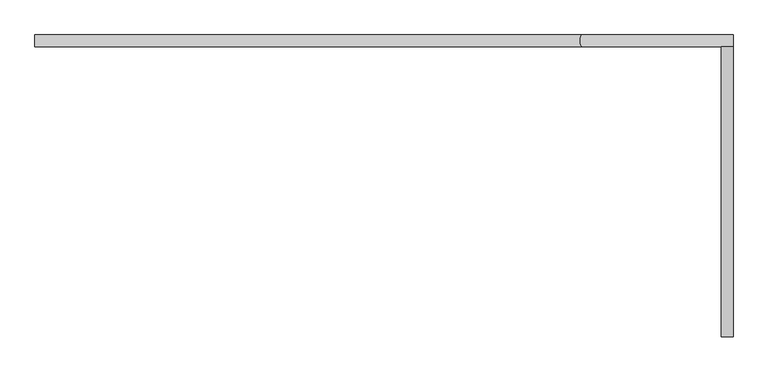
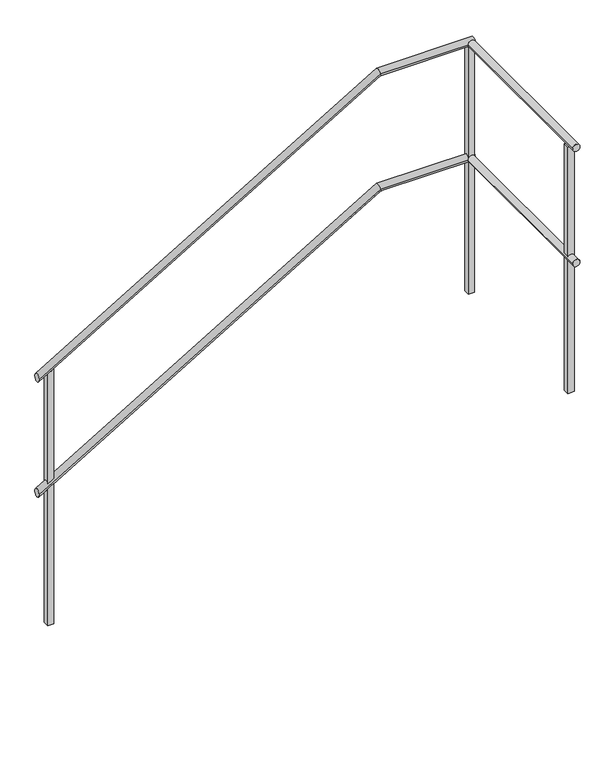
"""IFC4 building model written with IfcOpenShell, lengths in millimetres: railing geometry."""

from ifc_helpers import new_model, si_unit, frame, origin, place, context, project, spatial, polyline, circle_curve, ellipse_curve, outline, extrude, source, transform, mapped, element, save
from ifc_brep_helpers import plane_surface, cylinder_surface, advanced_brep


def railing_f6e22b08(model_context):
    return source(origin(), model_context, "Body", "SolidModel", [
        advanced_brep(
        [(43964.6, 23749.5208589, 1584.9618634), (43994.6, 23749.5208589, 1584.9618634), (43964.6, 24494.1208589, 1584.9618634), (43994.6, 24494.1208589, 1584.9618634)],
        [
            (0, 1, circle_curve(frame((43979.6, 23749.5208589, 1584.9618634), z_axis=(0.0, -1.0, 0.0), x_axis=(1.0, 0.0, 0.0)), 15.0)),
            (1, 0, circle_curve(frame((43979.6, 23749.5208589, 1584.9618634), z_axis=(0.0, -1.0, 0.0), x_axis=(1.0, 0.0, 0.0)), 15.0)),
            (2, 3, circle_curve(frame((43979.6, 24494.1208589, 1584.9618634), z_axis=(0.0, 1.0, 0.0), x_axis=(1.0, 0.0, 0.0)), 15.0)),
            (3, 2, circle_curve(frame((43979.6, 24494.1208589, 1584.9618634), z_axis=(0.0, 1.0, 0.0), x_axis=(1.0, 0.0, 0.0)), 15.0)),
            (0, 2),
            (3, 1),
        ],
        [
            plane_surface(frame((43979.6, 23749.5208589, 1599.9618634), z_axis=(0.0, -1.0, 0.0), x_axis=(0.0, 0.0, 1.0))),
            plane_surface(frame((43979.6, 24494.1208589, 1599.9618634), z_axis=(0.0, 1.0, 0.0), x_axis=(0.0, 0.0, 1.0))),
            cylinder_surface(frame((43979.6, 23749.5208589, 1584.9618634), z_axis=(0.0, -1.0, 0.0), x_axis=(1.0, 0.0, 0.0)), 15.0),
        ],
        [
            (0, [[1, 2]]),
            (1, [[3, 4]]),
            (2, [[-1, 5, -4, 6]]),
            (2, [[-2, -6, -3, -5]]),
        ],
    ),
        advanced_brep(
        [(43994.6, 24494.1208589, 1584.9618634), (43994.6, 24524.1208589, 1584.9618634), (43606.242552, 24494.1208589, 1584.9618634), (43606.242552, 24524.1208589, 1584.9618634), (42202.1161135, 24494.1208589, 749.1723166), (42202.1161135, 24524.1208589, 749.1723166)],
        [
            (0, 1, circle_curve(frame((43994.6, 24509.1208589, 1584.9618634), z_axis=(1.0, 0.0, 0.0), x_axis=(0.0, 1.0, 0.0)), 15.0)),
            (1, 0, circle_curve(frame((43994.6, 24509.1208589, 1584.9618634), z_axis=(1.0, 0.0, 0.0), x_axis=(0.0, 1.0, 0.0)), 15.0)),
            (0, 2),
            (2, 3, ellipse_curve(frame((43606.242552, 24509.1208589, 1584.9618634), z_axis=(0.9641817474962143, 0.0, 0.2652424509673111), x_axis=(0.265242450967311, 0.0, -0.9641817474962144)), 15.5572329, 15.0)),
            (3, 1),
            (3, 2, ellipse_curve(frame((43606.242552, 24509.1208589, 1584.9618634), z_axis=(0.9641817474962143, 0.0, 0.2652424509673111), x_axis=(0.265242450967311, 0.0, -0.9641817474962144)), 15.5572329, 15.0)),
            (4, 5, ellipse_curve(frame((42202.1161135, 24509.1208589, 749.1723166), z_axis=(-1.0, 0.0, 0.0), x_axis=(0.0, 0.0, 1.0)), 17.4562134, 15.0)),
            (5, 4, ellipse_curve(frame((42202.1161135, 24509.1208589, 749.1723166), z_axis=(-1.0, 0.0, 0.0), x_axis=(0.0, 0.0, 1.0)), 17.4562134, 15.0)),
            (2, 4),
            (5, 3),
        ],
        [
            plane_surface(frame((43994.6, 24509.1208589, 1599.9618634), z_axis=(1.0, 0.0, 0.0), x_axis=(0.0, -1.0, 0.0))),
            cylinder_surface(frame((43994.6, 24509.1208589, 1584.9618634), z_axis=(1.0, 0.0, 0.0), x_axis=(0.0, 1.0, 0.0)), 15.0),
            plane_surface(frame((42202.1161135, 24509.1208589, 766.62853), z_axis=(-1.0, 0.0, 0.0), x_axis=(0.0, -1.0, 0.0))),
            cylinder_surface(frame((43609.7883714, 24509.1208589, 1587.0724701), z_axis=(0.8592928844097072, 0.0, 0.5114838597676818), x_axis=(0.0, 1.0, 0.0)), 15.0),
        ],
        [
            (0, [[1, 2]]),
            (1, [[-1, 3, 4, 5]]),
            (1, [[-2, -5, 6, -3]]),
            (2, [[7, 8]]),
            (3, [[-4, 9, -8, 10]]),
            (3, [[-6, -10, -7, -9]]),
        ],
    ),
        advanced_brep(
        [(43964.6, 23749.5208589, 2084.9618634), (43994.6, 23749.5208589, 2084.9618634), (43964.6, 24494.1208589, 2084.9618634), (43994.6, 24494.1208589, 2084.9618634)],
        [
            (0, 1, circle_curve(frame((43979.6, 23749.5208589, 2084.9618634), z_axis=(0.0, -1.0, 0.0), x_axis=(1.0, 0.0, 0.0)), 15.0)),
            (1, 0, circle_curve(frame((43979.6, 23749.5208589, 2084.9618634), z_axis=(0.0, -1.0, 0.0), x_axis=(1.0, 0.0, 0.0)), 15.0)),
            (2, 3, circle_curve(frame((43979.6, 24494.1208589, 2084.9618634), z_axis=(0.0, 1.0, 0.0), x_axis=(1.0, 0.0, 0.0)), 15.0)),
            (3, 2, circle_curve(frame((43979.6, 24494.1208589, 2084.9618634), z_axis=(0.0, 1.0, 0.0), x_axis=(1.0, 0.0, 0.0)), 15.0)),
            (0, 2),
            (3, 1),
        ],
        [
            plane_surface(frame((43979.6, 23749.5208589, 2099.9618634), z_axis=(0.0, -1.0, 0.0), x_axis=(0.0, 0.0, 1.0))),
            plane_surface(frame((43979.6, 24494.1208589, 2099.9618634), z_axis=(0.0, 1.0, 0.0), x_axis=(0.0, 0.0, 1.0))),
            cylinder_surface(frame((43979.6, 23749.5208589, 2084.9618634), z_axis=(0.0, -1.0, 0.0), x_axis=(1.0, 0.0, 0.0)), 15.0),
        ],
        [
            (0, [[1, 2]]),
            (1, [[3, 4]]),
            (2, [[-1, 5, -4, 6]]),
            (2, [[-2, -6, -3, -5]]),
        ],
    ),
        advanced_brep(
        [(43994.6, 24494.1208589, 2084.9618634), (43994.6, 24524.1208589, 2084.9618634), (43606.242552, 24494.1208589, 2084.9618634), (43606.242552, 24524.1208589, 2084.9618634), (42202.1161135, 24494.1208589, 1249.1723166), (42202.1161135, 24524.1208589, 1249.1723166)],
        [
            (0, 1, circle_curve(frame((43994.6, 24509.1208589, 2084.9618634), z_axis=(1.0, 0.0, 0.0), x_axis=(0.0, 1.0, 0.0)), 15.0)),
            (1, 0, circle_curve(frame((43994.6, 24509.1208589, 2084.9618634), z_axis=(1.0, 0.0, 0.0), x_axis=(0.0, 1.0, 0.0)), 15.0)),
            (0, 2),
            (2, 3, ellipse_curve(frame((43606.242552, 24509.1208589, 2084.9618634), z_axis=(0.9641817474962143, 0.0, 0.2652424509673111), x_axis=(0.265242450967311, 0.0, -0.9641817474962144)), 15.5572329, 15.0)),
            (3, 1),
            (3, 2, ellipse_curve(frame((43606.242552, 24509.1208589, 2084.9618634), z_axis=(0.9641817474962143, 0.0, 0.2652424509673111), x_axis=(0.265242450967311, 0.0, -0.9641817474962144)), 15.5572329, 15.0)),
            (4, 5, ellipse_curve(frame((42202.1161135, 24509.1208589, 1249.1723166), z_axis=(-1.0, 0.0, 0.0), x_axis=(0.0, 0.0, 1.0)), 17.4562134, 15.0)),
            (5, 4, ellipse_curve(frame((42202.1161135, 24509.1208589, 1249.1723166), z_axis=(-1.0, 0.0, 0.0), x_axis=(0.0, 0.0, 1.0)), 17.4562134, 15.0)),
            (2, 4),
            (5, 3),
        ],
        [
            plane_surface(frame((43994.6, 24509.1208589, 2099.9618634), z_axis=(1.0, 0.0, 0.0), x_axis=(0.0, -1.0, 0.0))),
            cylinder_surface(frame((43994.6, 24509.1208589, 2084.9618634), z_axis=(1.0, 0.0, 0.0), x_axis=(0.0, 1.0, 0.0)), 15.0),
            plane_surface(frame((42202.1161135, 24509.1208589, 1266.62853), z_axis=(-1.0, 0.0, 0.0), x_axis=(0.0, -1.0, 0.0))),
            cylinder_surface(frame((43609.7883714, 24509.1208589, 2087.0724701), z_axis=(0.8592928844097072, 0.0, 0.5114838597676818), x_axis=(0.0, 1.0, 0.0)), 15.0),
        ],
        [
            (0, [[1, 2]]),
            (1, [[-1, 3, 4, 5]]),
            (1, [[-2, -5, 6, -3]]),
            (2, [[7, 8]]),
            (3, [[-4, 9, -8, 10]]),
            (3, [[-6, -10, -7, -9]]),
        ],
    ),
        extrude(outline(polyline([(43992.1, 24496.6208589), (43967.1, 24496.6208589), (43967.1, 24521.6208589), (43992.1, 24521.6208589), (43992.1, 24496.6208589)])), frame((0.0, 0.0, 999.9618634), z_axis=(0.0, 0.0, 1.0), x_axis=(1.0, 0.0, 0.0)), (0.0, 0.0, 1.0), 1070.0),
        extrude(outline(polyline([(166.62853, 42264.6161135), (1273.830911, 42264.6161135), (1258.9499586, 42239.6161135), (166.62853, 42239.6161135), (166.62853, 42264.6161135)])), frame((0.0, 24496.6208589, 0.0), z_axis=(0.0, 1.0, 0.0), x_axis=(0.0, 0.0, 1.0)), (0.0, 0.0, 1.0), 25.0),
        extrude(outline(polyline([(43992.1, 23787.0208589), (43967.1, 23787.0208589), (43967.1, 23812.0208589), (43992.1, 23812.0208589), (43992.1, 23787.0208589)])), frame((0.0, 0.0, 999.9618634), z_axis=(0.0, 0.0, 1.0), x_axis=(1.0, 0.0, 0.0)), (0.0, 0.0, 1.0), 1070.0),
    ])


if __name__ == "__main__":
    model = new_model("IFC4")
    model_context = context("Model", 3, world=origin())
    ifc_project = project(units=[si_unit("LENGTHUNIT", "METRE", prefix="MILLI")], contexts=[model_context])
    site = spatial("IfcSite", under=ifc_project)
    building = spatial("IfcBuilding", under=site)
    placement = place(None, origin())
    railing_shape = railing_f6e22b08(model_context)
    element("IfcRailing", 1, at=placement, inside=building, context=model_context, shape_type="MappedRepresentation", body=[
        mapped(railing_shape, transform((0.0, 0.0, 0.0), x_axis=(1.0, 0.0, 0.0), y_axis=(0.0, 1.0, 0.0), z_axis=(0.0, 0.0, 1.0))),
    ])
    save(model, "model.ifc")
